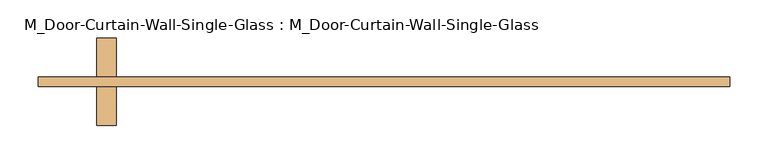
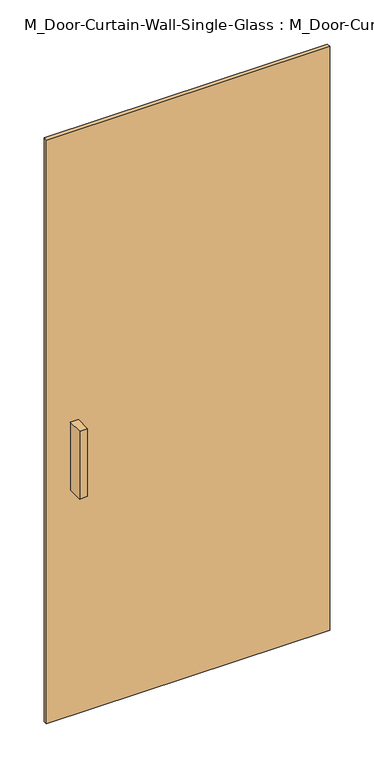
"""IFC4 building model written with IfcOpenShell, lengths in millimetres: door geometry, M_Door-Curtain-Wall-Single-Glass : M_Door-Curtain-Wall-Single-Glass."""

from ifc_helpers import new_model, si_unit, frame, origin, origin_with_axes, place, context, project, spatial, polyline, outline, extrude, source, transform, mapped, element, save


def m_door_curtain_wall_single_glass_m_door_curtain_wall_single_b3f25844(model_context):
    return source(origin(), model_context, "Body", "SweptSolid", [
        extrude(outline(polyline([(451.2499998, 50.8), (451.2499998, 38.1), (-451.2499998, 38.1), (-451.2499998, 50.8), (451.2499998, 50.8)])), origin_with_axes(), (0.0, 0.0, 1.0), 1967.5),
        extrude(outline(polyline([(-375.0499998, 101.6), (-349.6499998, 101.6), (-349.6499998, 50.8), (-375.0499998, 50.8), (-375.0499998, 101.6)])), frame((0.0, 0.0, 762.0), z_axis=(0.0, 0.0, 1.0), x_axis=(1.0, 0.0, 0.0)), (0.0, 0.0, 1.0), 228.6),
        extrude(outline(polyline([(-349.6499998, -12.7), (-375.0499998, -12.7), (-375.0499998, 38.1), (-349.6499998, 38.1), (-349.6499998, -12.7)])), frame((0.0, 0.0, 762.0), z_axis=(0.0, 0.0, 1.0), x_axis=(1.0, 0.0, 0.0)), (0.0, 0.0, 1.0), 228.6),
    ])


if __name__ == "__main__":
    model = new_model("IFC4")
    model_context = context("Model", 3, world=origin())
    ifc_project = project(units=[si_unit("LENGTHUNIT", "METRE", prefix="MILLI")], contexts=[model_context])
    site = spatial("IfcSite", under=ifc_project)
    building = spatial("IfcBuilding", under=site)
    placement = place(None, origin())
    m_door_curtain_wall_single_glass_m_door_curtain_wall_single_shape = m_door_curtain_wall_single_glass_m_door_curtain_wall_single_b3f25844(model_context)
    element("IfcDoor", 1, ObjectType="M_Door-Curtain-Wall-Single-Glass : M_Door-Curtain-Wall-Single-Glass", at=placement, inside=building, context=model_context, shape_type="MappedRepresentation", body=[
        mapped(m_door_curtain_wall_single_glass_m_door_curtain_wall_single_shape, transform((0.0, 0.0, 0.0), x_axis=(1.0, 0.0, 0.0), y_axis=(0.0, 1.0, 0.0), z_axis=(0.0, 0.0, 1.0))),
    ])
    save(model, "model.ifc")

# Revit data of these elements
# Type "M_Door-Curtain-Wall-Single-Glass : M_Door-Curtain-Wall-Single-Glass"
#   Type Mark = "D-49"
#   Assembly Code = "B2030100"
#   Analytic Construction = "<None>"
#   Width [instance default] = 0.900 m
#   Thermal Resistance (R) = 1.7611 (m²·K)/W
#   Swing Angle [instance default] = 90.00°
#   Heat Transfer Coefficient (U) = 0.567826 W/(m²·K)
#   Offset = 0.0508 m
#   Define Thermal Properties by = 1
#   Function = 1
#   Door Handle Material = Aluminum
#   Glazing = Glass
#   Visual Light Transmittance = 0
#   Solar Heat Gain Coefficient = 0
#   Construction Type Id = ""
# Element 1 (IfcDoor, "M_Door-Curtain-Wall-Single-Glass : M_Door-Curtain-Wall-Single-Glass")
#   Width = 0.9025 m
#   Materials on its faces: "Aluminum", "Glass"
# Materials
#   "Aluminum": class "Metal", colour RGB 244 245 246, transparency 0, Description = "Aluminum 6061", Cost = 0
#   "Glass": class "Glass", colour RGB 245 245 243, transparency 1, Description = "Soda Lime Glass", Cost = 0
